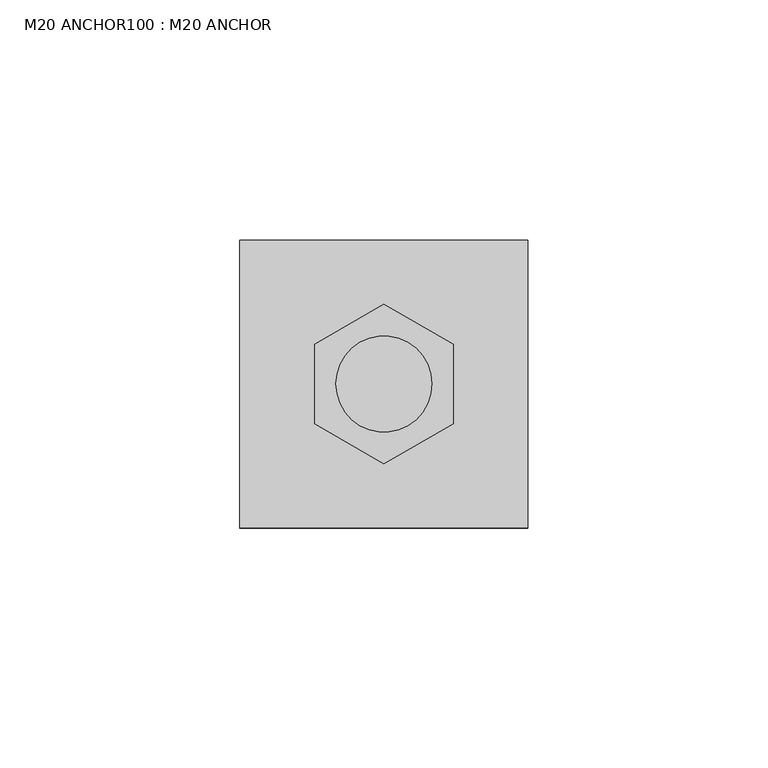
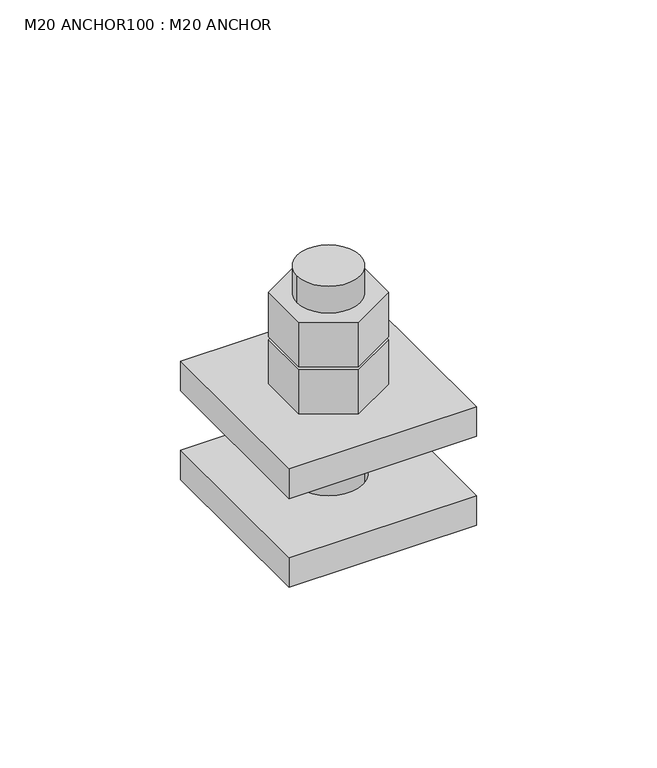
"""IFC4 building model written with IfcOpenShell, lengths in millimetres: fastener geometry, M20 ANCHOR100 : M20 ANCHOR."""

from ifc_helpers import new_model, si_unit, point, frame, frame_2d, origin, place, context, project, spatial, polyline, circle_curve, trimmed, segment, composite_curve, outline, extrude, source, transform, mapped, element, save


def m20_anchor100_m20_anchor_ca884006(model_context):
    return source(origin(), model_context, "Body", "SweptSolid", [
        extrude(outline(polyline([(15008.0855968, 22453.9464399), (15008.0855968, 22470.5835027), (15022.4937158, 22478.9020341), (15036.9018348, 22470.5835027), (15036.9018348, 22453.9464399), (15022.4937158, 22445.6279085), (15008.0855968, 22453.9464399)]), holes=[composite_curve([segment(trimmed(circle_curve(frame_2d((15022.4937158, 22462.2649713)), 10.0), [point((15032.4937158, 22462.2649713))], [point((15012.4937158, 22462.2649713))], True, "CARTESIAN"), True, "CONTINUOUS"), segment(trimmed(circle_curve(frame_2d((15022.4937158, 22462.2649713)), 10.0), [point((15012.4937158, 22462.2649713))], [point((15032.4937158, 22462.2649713))], True, "CARTESIAN"), True, "CONTINUOUS")], self_intersect=False)]), frame((0.0, 0.0, 246.0), z_axis=(0.0, 0.0, 1.0), x_axis=(1.0, 0.0, 0.0)), (0.0, 0.0, 1.0), 15.0),
        extrude(outline(polyline([(15008.0855968, 22453.9464399), (15008.0855968, 22470.5835027), (15022.4937158, 22478.9020341), (15036.9018348, 22470.5835027), (15036.9018348, 22453.9464399), (15022.4937158, 22445.6279085), (15008.0855968, 22453.9464399)]), holes=[composite_curve([segment(trimmed(circle_curve(frame_2d((15022.4937158, 22462.2649713)), 10.0), [point((15032.4937158, 22462.2649713))], [point((15012.4937158, 22462.2649713))], True, "CARTESIAN"), True, "CONTINUOUS"), segment(trimmed(circle_curve(frame_2d((15022.4937158, 22462.2649713)), 10.0), [point((15012.4937158, 22462.2649713))], [point((15032.4937158, 22462.2649713))], True, "CARTESIAN"), True, "CONTINUOUS")], self_intersect=False)]), frame((0.0, 0.0, 230.0), z_axis=(0.0, 0.0, 1.0), x_axis=(1.0, 0.0, 0.0)), (0.0, 0.0, 1.0), 15.0),
        extrude(outline(composite_curve([segment(trimmed(circle_curve(frame_2d((15022.4937158, 22462.2649713)), 10.0), [point((15032.4937158, 22462.2649713))], [point((15012.4937158, 22462.2649713))], False, "CARTESIAN"), True, "CONTINUOUS"), segment(trimmed(circle_curve(frame_2d((15022.4937158, 22462.2649713)), 10.0), [point((15012.4937158, 22462.2649713))], [point((15032.4937158, 22462.2649713))], False, "CARTESIAN"), True, "CONTINUOUS")], self_intersect=False)), frame((0.0, 0.0, 190.0), z_axis=(0.0, 0.0, 1.0), x_axis=(1.0, 0.0, 0.0)), (0.0, 0.0, 1.0), 80.0),
        extrude(outline(polyline([(14992.4937158, 22432.2649713), (14992.4937158, 22492.2649713), (15052.4937158, 22492.2649713), (15052.4937158, 22432.2649713), (14992.4937158, 22432.2649713)]), holes=[composite_curve([segment(trimmed(circle_curve(frame_2d((15022.4937158, 22462.2649713)), 11.0), [point((15033.4937158, 22462.2649713))], [point((15011.4937158, 22462.2649713))], True, "CARTESIAN"), True, "CONTINUOUS"), segment(trimmed(circle_curve(frame_2d((15022.4937158, 22462.2649713)), 11.0), [point((15011.4937158, 22462.2649713))], [point((15033.4937158, 22462.2649713))], True, "CARTESIAN"), True, "CONTINUOUS")], self_intersect=False)]), frame((0.0, 0.0, 190.0), z_axis=(0.0, 0.0, 1.0), x_axis=(1.0, 0.0, 0.0)), (0.0, 0.0, 1.0), 10.0),
        extrude(outline(polyline([(14992.4937158, 22432.2649713), (14992.4937158, 22492.2649713), (15052.4937158, 22492.2649713), (15052.4937158, 22432.2649713), (14992.4937158, 22432.2649713)]), holes=[composite_curve([segment(trimmed(circle_curve(frame_2d((15022.4937158, 22462.2649713)), 11.0), [point((15033.4937158, 22462.2649713))], [point((15011.4937158, 22462.2649713))], True, "CARTESIAN"), True, "CONTINUOUS"), segment(trimmed(circle_curve(frame_2d((15022.4937158, 22462.2649713)), 11.0), [point((15011.4937158, 22462.2649713))], [point((15033.4937158, 22462.2649713))], True, "CARTESIAN"), True, "CONTINUOUS")], self_intersect=False)]), frame((0.0, 0.0, 220.0), z_axis=(0.0, 0.0, 1.0), x_axis=(1.0, 0.0, 0.0)), (0.0, 0.0, 1.0), 10.0),
    ])


if __name__ == "__main__":
    model = new_model("IFC4")
    model_context = context("Model", 3, world=origin())
    ifc_project = project(units=[si_unit("LENGTHUNIT", "METRE", prefix="MILLI")], contexts=[model_context])
    site = spatial("IfcSite", under=ifc_project)
    building = spatial("IfcBuilding", under=site)
    placement = place(None, origin())
    m20_anchor100_m20_anchor_shape = m20_anchor100_m20_anchor_ca884006(model_context)
    element("IfcFastener", 1, ObjectType="M20 ANCHOR100 : M20 ANCHOR", at=placement, inside=building, context=model_context, shape_type="MappedRepresentation", body=[
        mapped(m20_anchor100_m20_anchor_shape, transform((0.0, 0.0, 0.0), x_axis=(1.0, 0.0, 0.0), y_axis=(0.0, 1.0, 0.0), z_axis=(0.0, 0.0, 1.0))),
    ])
    save(model, "model.ifc")
